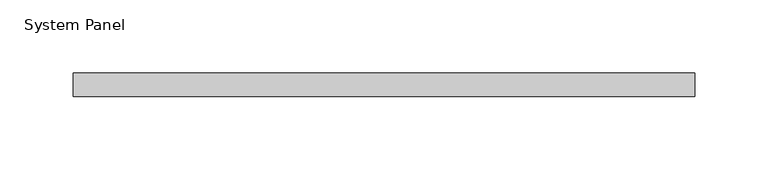
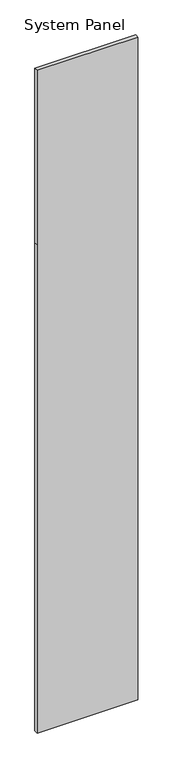
"""IFC4 building model written with IfcOpenShell, lengths in millimetres: plate geometry, System Panel : 로이복층유리_16."""

from ifc_helpers import new_model, si_unit, frame, origin, place, context, project, spatial, polyline, outline, extrude, source, transform, mapped, element, save


def system_panel_3b38218c(model_context):
    return source(origin(), model_context, "Body", "SweptSolid", [
        extrude(outline(polyline([(0.0, -212.5), (0.0, 212.5), (2177.5, 212.5), (2955.0, 212.5), (2955.0, -212.5), (2177.5, -212.5), (0.0, -212.5)])), frame((0.0, -8.0, 0.0), z_axis=(0.0, 1.0, 0.0), x_axis=(0.0, 0.0, 1.0)), (0.0, 0.0, 1.0), 16.0),
    ])


if __name__ == "__main__":
    model = new_model("IFC4")
    model_context = context("Model", 3, world=origin())
    ifc_project = project(units=[si_unit("LENGTHUNIT", "METRE", prefix="MILLI")], contexts=[model_context])
    site = spatial("IfcSite", under=ifc_project)
    building = spatial("IfcBuilding", under=site)
    placement = place(None, origin())
    system_panel_shape = system_panel_3b38218c(model_context)
    element("IfcPlate", 1, ObjectType="System Panel : 로이복층유리_16", at=placement, inside=building, context=model_context, shape_type="MappedRepresentation", body=[
        mapped(system_panel_shape, transform((0.0, 0.0, 0.0), x_axis=(1.0, 0.0, 0.0), y_axis=(0.0, 1.0, 0.0), z_axis=(0.0, 0.0, 1.0))),
    ])
    save(model, "model.ifc")

# Revit data of these elements
# Element 1 (IfcPlate, "System Panel : 로이복층유리_16")
#   Materials on its faces: "00_Glass_Glass"
# Materials
#   "00_Glass_Glass": class "Glass", colour RGB 218 227 224, transparency 0.85, Description = "Glass", Cost = 0, Image = none
